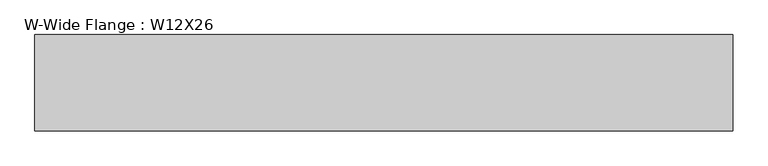
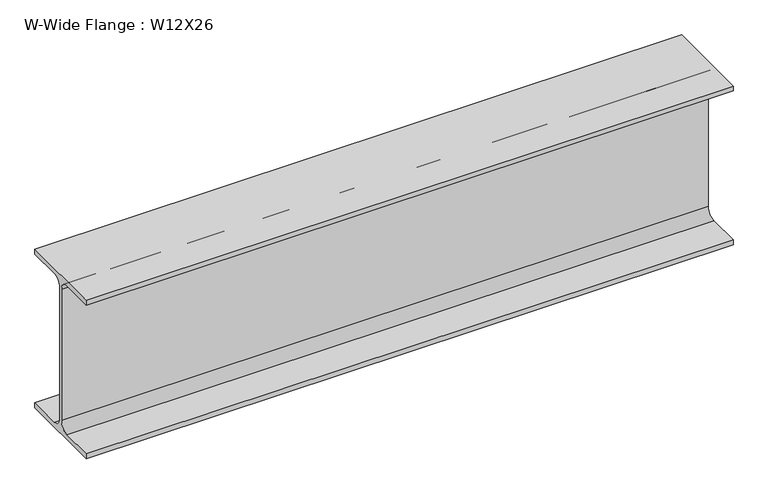
"""IFC4 building model written with IfcOpenShell, lengths in millimetres: beam geometry, W-Wide Flange : W12X26."""

from ifc_helpers import new_model, si_unit, point, frame, frame_2d, origin, place, context, project, spatial, polyline, circle_curve, trimmed, segment, composite_curve, outline, extrude, source, transform, mapped, element, save


def w_wide_flange_w12x26_b418ac95(model_context):
    return source(origin(), model_context, "Body", "SweptSolid", [
        extrude(outline(composite_curve([segment(polyline([(82.4011719, -145.5539063), (82.4011719, -155.178125), (-82.4011719, -155.178125), (-82.4011719, -145.5539063), (-20.2902344, -145.5539063)]), True, "CONTINUOUS"), segment(trimmed(circle_curve(frame_2d((-20.2902344, -128.190625)), 17.3632812), [point((-20.2902344, -145.5539063))], [point((-2.9269531, -128.190625))], True, "CARTESIAN"), True, "CONTINUOUS"), segment(polyline([(-2.9269531, -128.190625), (-2.9269531, 128.190625)]), True, "CONTINUOUS"), segment(trimmed(circle_curve(frame_2d((-20.2902344, 128.190625)), 17.3632812), [point((-2.9269531, 128.190625))], [point((-20.2902344, 145.5539062))], True, "CARTESIAN"), True, "CONTINUOUS"), segment(polyline([(-20.2902344, 145.5539062), (-82.4011719, 145.5539062), (-82.4011719, 155.178125), (82.4011719, 155.178125), (82.4011719, 145.5539062), (20.2902344, 145.5539062)]), True, "CONTINUOUS"), segment(trimmed(circle_curve(frame_2d((20.2902344, 128.190625)), 17.3632812), [point((20.2902344, 145.5539062))], [point((2.9269531, 128.190625))], True, "CARTESIAN"), True, "CONTINUOUS"), segment(polyline([(2.9269531, 128.190625), (2.9269531, -128.190625)]), True, "CONTINUOUS"), segment(trimmed(circle_curve(frame_2d((20.2902344, -128.190625)), 17.3632812), [point((2.9269531, -128.190625))], [point((20.2902344, -145.5539063))], True, "CARTESIAN"), True, "CONTINUOUS"), segment(polyline([(20.2902344, -145.5539063), (82.4011719, -145.5539063)]), True, "CONTINUOUS")], self_intersect=False)), frame((-639.4520065, 0.0, 0.0), z_axis=(1.0, 0.0, 0.0), x_axis=(0.0, 1.0, 0.0)), (0.0, 0.0, 1.0), 1196.5028412),
    ])


if __name__ == "__main__":
    model = new_model("IFC4")
    model_context = context("Model", 3, world=origin())
    ifc_project = project(units=[si_unit("LENGTHUNIT", "METRE", prefix="MILLI")], contexts=[model_context])
    site = spatial("IfcSite", under=ifc_project)
    building = spatial("IfcBuilding", under=site)
    placement = place(None, origin())
    w_wide_flange_w12x26_shape = w_wide_flange_w12x26_b418ac95(model_context)
    element("IfcBeam", 1, ObjectType="W-Wide Flange : W12X26", at=placement, inside=building, context=model_context, shape_type="MappedRepresentation", body=[
        mapped(w_wide_flange_w12x26_shape, transform((0.0, 0.0, 0.0), x_axis=(1.0, 0.0, 0.0), y_axis=(0.0, 1.0, 0.0), z_axis=(0.0, 0.0, 1.0))),
    ])
    save(model, "model.ifc")

# Revit data of these elements
# Type "W-Wide Flange : W12X26"
#   Assembly Code = "B10"
#   W = 26
#   Length [instance default] = 5' - 0"
#   bf = 0' - 6 125/256"
#   d = 1' - 0 7/32"
#   k = 0' - 1 1/16"
#   k2 = 0' - 0 175/256"
#   tf = 0' - 0 97/256"
#   tw = 0' - 0 59/256"
#   A = 0.053125 SF
#   Structural Material [instance default] = none
# Element 1 (IfcBeam, "W-Wide Flange : W12X26")
#   Structural Material = Dark metal
#   Materials on its faces: "Dark metal"
# Materials
#   "Dark metal": class "Generic", colour RGB 44 29 29, transparency 0, Cost = 0
